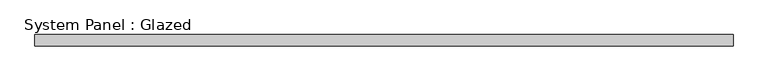
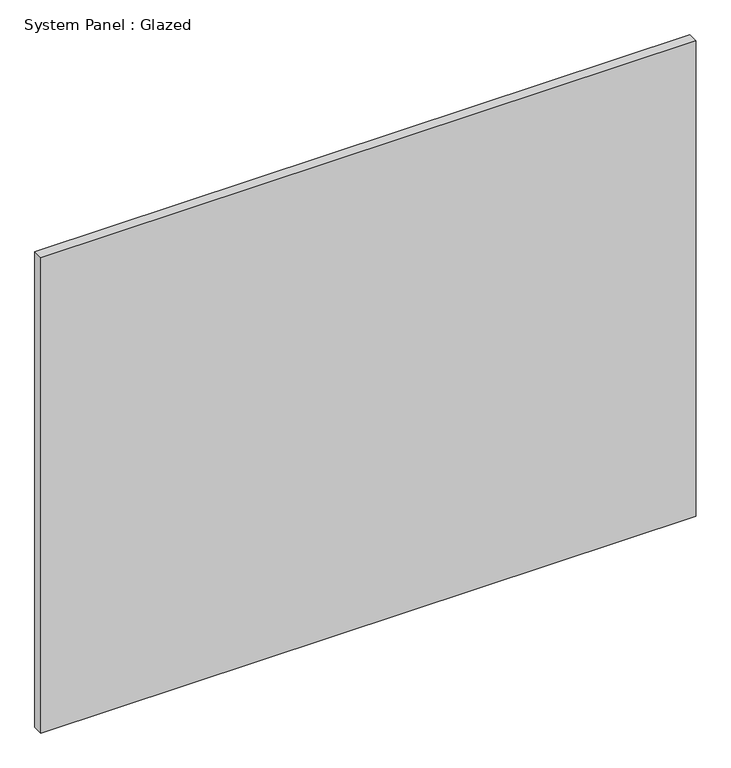
"""IFC4 building model written with IfcOpenShell, lengths in millimetres: plate geometry, System Panel : Glazed."""

from ifc_helpers import new_model, si_unit, origin, origin_with_axes, place, context, project, spatial, polyline, outline, extrude, source, transform, mapped, element, save


def system_panel_glazed_f2fc581d(model_context):
    return source(origin(), model_context, "Body", "SweptSolid", [
        extrude(outline(polyline([(782.9080161, 24.5), (-782.9080161, 24.5), (-782.9080161, 49.5), (782.9080161, 49.5), (782.9080161, 24.5)])), origin_with_axes(), (0.0, 0.0, 1.0), 1200.0),
    ])


if __name__ == "__main__":
    model = new_model("IFC4")
    model_context = context("Model", 3, world=origin())
    ifc_project = project(units=[si_unit("LENGTHUNIT", "METRE", prefix="MILLI")], contexts=[model_context])
    site = spatial("IfcSite", under=ifc_project)
    building = spatial("IfcBuilding", under=site)
    placement = place(None, origin())
    system_panel_glazed_shape = system_panel_glazed_f2fc581d(model_context)
    element("IfcPlate", 1, ObjectType="System Panel : Glazed", at=placement, inside=building, context=model_context, shape_type="MappedRepresentation", body=[
        mapped(system_panel_glazed_shape, transform((0.0, 0.0, 0.0), x_axis=(1.0, 0.0, 0.0), y_axis=(0.0, 1.0, 0.0), z_axis=(0.0, 0.0, 1.0))),
    ])
    save(model, "model.ifc")

# Revit data of these elements
# Element 1 (IfcPlate, "System Panel : Glazed")
#   Materials on its faces: "Glass"
# Materials
#   "Glass": class "Glass", colour RGB 218 227 224, transparency 0.85, Description = "Soda Lime Glass", Cost = 0
